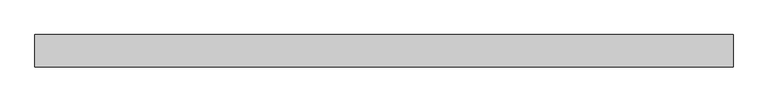
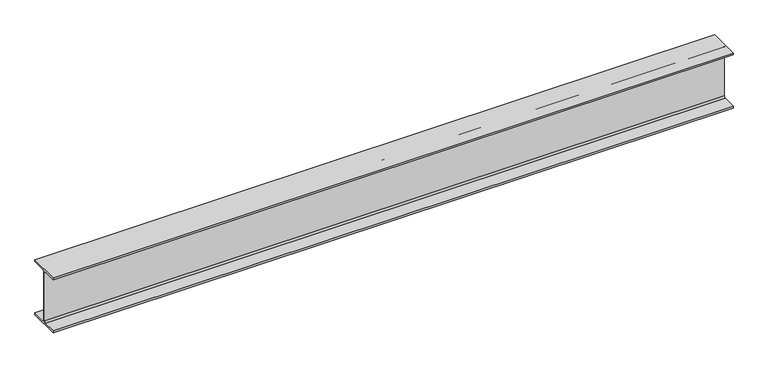
"""IFC4 building model written with IfcOpenShell, lengths in millimetres: beam geometry, Old_Steel Beam_H-KSD3502 : H_SB_ASB_H-200×200x8x12."""

import ifcopenshell
import ifcopenshell.guid

model = None  # the IFC model being written
_history = None  # IfcOwnerHistory: only IFC2X3 demands one
_inside = {}  # id of a spatial element -> (the spatial element, [elements in it])
_under = {}  # id of a project, library or spatial element -> (it, [spatial elements below it])
_declared = {}  # id of a project -> (the project, [libraries it declares])
_typed = {}  # id of a type object -> (the type object, [elements of that type])
_made_of = {}  # id of a material, layer set ... -> (it, [elements and type objects made of it])


def new_model(schema):
    """Start an empty IFC model of exactly this schema.

    Asked for "IFC4X3", IfcOpenShell would pick the latest addendum, in which some entities
    have other attributes; the version numbers below select the first issue.
    IFC2X3 requires an IfcOwnerHistory on every rooted entity: one is made here for all.
    """
    global model, _history
    if schema == "IFC4X3":
        model = ifcopenshell.file(schema_version=(4, 3, 0, 0))
    else:
        model = ifcopenshell.file(schema=schema)
    _inside.clear()
    _under.clear()
    _declared.clear()
    _typed.clear()
    _made_of.clear()
    _history = None
    if model.schema == "IFC2X3":
        org = make("IfcOrganization", Name="unknown")
        user = make(
            "IfcPersonAndOrganization",
            ThePerson=make("IfcPerson", FamilyName="unknown"),
            TheOrganization=org,
        )
        app = make(
            "IfcApplication",
            ApplicationDeveloper=org,
            Version="unknown",
            ApplicationFullName="unknown",
            ApplicationIdentifier="unknown",
        )
        _history = make(
            "IfcOwnerHistory",
            OwningUser=user,
            OwningApplication=app,
            ChangeAction="ADDED",
            CreationDate=0,
        )
    return model


def make(cls, **values):
    """One entity of the class cls with the attributes given. An attribute that is None is left unset."""
    return model.create_entity(
        cls, **{name: value for name, value in values.items() if value is not None}
    )


def rooted(cls, **values):
    """An entity with a GlobalId (a new one), such as an element, a storey or a relation."""
    return make(cls, GlobalId=ifcopenshell.guid.new(), OwnerHistory=_history, **values)


def si_unit(unit_type, name, prefix=None):
    """IfcSIUnit, for example si_unit("LENGTHUNIT", "METRE", prefix="MILLI")."""
    return make("IfcSIUnit", UnitType=unit_type, Prefix=prefix, Name=name)


def assignment(units):
    """IfcUnitAssignment: the units of a project."""
    return None if units is None else make("IfcUnitAssignment", Units=units)


def point(xyz):
    """IfcCartesianPoint."""
    return None if xyz is None else make("IfcCartesianPoint", Coordinates=xyz)


def direction(xyz):
    """IfcDirection."""
    return None if xyz is None else make("IfcDirection", DirectionRatios=xyz)


def frame(location, z_axis=None, x_axis=None):
    """IfcAxis2Placement3D, a coordinate frame: its origin and axes. An axis left out is left unset."""
    return make(
        "IfcAxis2Placement3D",
        Location=point(location),
        Axis=direction(z_axis),
        RefDirection=direction(x_axis),
    )


def frame_2d(location, x_axis=None):
    """IfcAxis2Placement2D, a coordinate frame in the plane: its origin and x axis."""
    return make(
        "IfcAxis2Placement2D", Location=point(location), RefDirection=direction(x_axis)
    )


def origin():
    """The frame at (0, 0, 0) with its axes left unset."""
    return frame((0.0, 0.0, 0.0))


def place(relative_to, where):
    """IfcLocalPlacement: puts the frame where relative to a parent placement (None: the world)."""
    return make(
        "IfcLocalPlacement", PlacementRelTo=relative_to, RelativePlacement=where
    )


def context(
    kind, dimensions, precision=None, world=None, true_north=None, identifier=None
):
    """IfcGeometricRepresentationContext, for example the 3D "Model" context."""
    return make(
        "IfcGeometricRepresentationContext",
        ContextIdentifier=identifier,
        ContextType=kind,
        CoordinateSpaceDimension=dimensions,
        Precision=precision,
        WorldCoordinateSystem=world,
        TrueNorth=true_north,
    )


def project(units=None, contexts=None):
    """IfcProject with its units and contexts."""
    return rooted(
        "IfcProject",
        Name="project",
        RepresentationContexts=contexts,
        UnitsInContext=assignment(units),
    )


def spatial(cls, under=None, at=None, **own):
    """A site, building, storey or space (cls), placed at a placement, below another one or the project."""
    s = rooted(cls, ObjectPlacement=at, **own)
    if under is not None:
        _under.setdefault(under.id(), (under, []))[1].append(s)
    return s


def polyline(points):
    """IfcPolyline through the points."""
    return make("IfcPolyline", Points=[point(p) for p in points])


def circle_curve(where, radius):
    """IfcCircle in the frame where."""
    return make("IfcCircle", Position=where, Radius=radius)


def trimmed(basis, trim1, trim2, sense, master):
    """IfcTrimmedCurve: the piece of a basis curve between two trims."""
    return make(
        "IfcTrimmedCurve",
        BasisCurve=basis,
        Trim1=trim1,
        Trim2=trim2,
        SenseAgreement=sense,
        MasterRepresentation=master,
    )


def segment(curve, same_sense, transition):
    """IfcCompositeCurveSegment."""
    return make(
        "IfcCompositeCurveSegment",
        Transition=transition,
        SameSense=same_sense,
        ParentCurve=curve,
    )


def composite_curve(segments, self_intersect=None):
    """IfcCompositeCurve: segments joined end to end."""
    return make("IfcCompositeCurve", Segments=segments, SelfIntersect=self_intersect)


def outline(outer, holes=None, kind="AREA"):
    """IfcArbitraryClosedProfileDef: a profile drawn as a closed curve; with holes, ...WithVoids."""
    if holes is None:
        return make("IfcArbitraryClosedProfileDef", ProfileType=kind, OuterCurve=outer)
    return make(
        "IfcArbitraryProfileDefWithVoids",
        ProfileType=kind,
        OuterCurve=outer,
        InnerCurves=holes,
    )


def extrude(swept, where, along, depth):
    """IfcExtrudedAreaSolid: the profile swept, set in the frame where, extruded along a direction by depth."""
    return make(
        "IfcExtrudedAreaSolid",
        SweptArea=swept,
        Position=where,
        ExtrudedDirection=direction(along),
        Depth=depth,
    )


def shape(context_of_items, identifier, shape_type, items):
    """IfcShapeRepresentation: the items that make up one representation, for example the "Body"."""
    return make(
        "IfcShapeRepresentation",
        ContextOfItems=context_of_items,
        RepresentationIdentifier=identifier,
        RepresentationType=shape_type,
        Items=items,
    )


def source(mapping_origin, context_of_items, identifier, shape_type, items):
    """IfcRepresentationMap: a shape defined once, which mapped items show again and again."""
    return make(
        "IfcRepresentationMap",
        MappingOrigin=mapping_origin,
        MappedRepresentation=shape(context_of_items, identifier, shape_type, items),
    )


def transform(
    local_origin,
    x_axis=None,
    y_axis=None,
    z_axis=None,
    scale=None,
    scale2=None,
    scale3=None,
    uniform=True,
):
    """IfcCartesianTransformationOperator3D, or its non-uniform kind. x_axis, y_axis, z_axis: its Axis1, 2, 3."""
    if uniform:
        return make(
            "IfcCartesianTransformationOperator3D",
            Axis1=direction(x_axis),
            Axis2=direction(y_axis),
            LocalOrigin=point(local_origin),
            Scale=scale,
            Axis3=direction(z_axis),
        )
    return make(
        "IfcCartesianTransformationOperator3DnonUniform",
        Axis1=direction(x_axis),
        Axis2=direction(y_axis),
        LocalOrigin=point(local_origin),
        Scale=scale,
        Axis3=direction(z_axis),
        Scale2=scale2,
        Scale3=scale3,
    )


def mapped(mapping_source, mapping_target):
    """IfcMappedItem: shows the shape of a source again, moved by a transform."""
    return make(
        "IfcMappedItem", MappingSource=mapping_source, MappingTarget=mapping_target
    )


def made_of(thing, what):
    """Note that an element or type object is made of a material, layer set ...; save() writes the relation."""
    if what is not None:
        _made_of.setdefault(what.id(), (what, []))[1].append(thing)
    return thing


def element(
    cls,
    number,
    at=None,
    inside=None,
    cuts=None,
    type_object=None,
    material=None,
    context=None,
    identifier="Body",
    shape_type=None,
    held_by="IfcProductDefinitionShape",
    body=None,
    shapes=None,
    **own,
):
    """One element of the class cls, such as IfcWall. Its Tag is "e" and its number.

    at: its placement. inside: the storey or other place that contains it. cuts: it is an
    opening in that element (IfcRelVoidsElement). A single representation is given by context,
    identifier, shape_type and body (its items); several are given by shapes. held_by: the class
    of the entity that holds the representations. save() writes the other relations.
    """
    e = rooted(cls, Tag="e%d" % number, ObjectPlacement=at, **own)
    if body is not None:
        shapes = [shape(context, identifier, shape_type, body)]
    if shapes is not None:
        e.Representation = make(held_by, Representations=shapes)
    if inside is not None:
        _inside.setdefault(inside.id(), (inside, []))[1].append(e)
    if cuts is not None:
        rooted(
            "IfcRelVoidsElement", RelatingBuildingElement=cuts, RelatedOpeningElement=e
        )
    if type_object is not None:
        _typed.setdefault(type_object.id(), (type_object, []))[1].append(e)
    return made_of(e, material)


def aggregate(whole, parts):
    """IfcRelAggregates: a whole, such as a stair, and the parts it consists of."""
    return rooted("IfcRelAggregates", RelatingObject=whole, RelatedObjects=parts)


def save(model, path):
    """Write the relations noted so far, then the file.

    IfcRelAggregates (storeys below a building ...), IfcRelContainedInSpatialStructure (elements
    in a storey), IfcRelDefinesByType, IfcRelAssociatesMaterial and IfcRelDeclares: one each for
    every whole, place, type object, material and project.
    """
    for whole, parts in _under.values():
        aggregate(whole, parts)
    for where, things in _inside.values():
        rooted(
            "IfcRelContainedInSpatialStructure",
            RelatedElements=things,
            RelatingStructure=where,
        )
    for kind, things in _typed.values():
        rooted("IfcRelDefinesByType", RelatedObjects=things, RelatingType=kind)
    for what, things in _made_of.values():
        rooted("IfcRelAssociatesMaterial", RelatedObjects=things, RelatingMaterial=what)
    for by, libraries in _declared.values():
        rooted("IfcRelDeclares", RelatingContext=by, RelatedDefinitions=libraries)
    model.write(path)


def beam_588beb59(model_context):
    return source(origin(), model_context, "Body", "SweptSolid", [
        extrude(outline(composite_curve([segment(polyline([(82.5, -141.5), (82.5, -151.7), (-82.5, -151.7), (-82.5, -141.5), (-11.9, -141.5)]), True, "CONTINUOUS"), segment(trimmed(circle_curve(frame_2d((-11.9, -132.6)), 8.9), [point((-11.9, -141.5))], [point((-3.0, -132.6))], True, "CARTESIAN"), True, "CONTINUOUS"), segment(polyline([(-3.0, -132.6), (-3.0, 132.6)]), True, "CONTINUOUS"), segment(trimmed(circle_curve(frame_2d((-11.9, 132.6)), 8.9), [point((-3.0, 132.6))], [point((-11.9, 141.5))], True, "CARTESIAN"), True, "CONTINUOUS"), segment(polyline([(-11.9, 141.5), (-82.5, 141.5), (-82.5, 151.7), (82.5, 151.7), (82.5, 141.5), (11.9, 141.5)]), True, "CONTINUOUS"), segment(trimmed(circle_curve(frame_2d((11.9, 132.6)), 8.9), [point((11.9, 141.5))], [point((3.0, 132.6))], True, "CARTESIAN"), True, "CONTINUOUS"), segment(polyline([(3.0, 132.6), (3.0, -132.6)]), True, "CONTINUOUS"), segment(trimmed(circle_curve(frame_2d((11.9, -132.6)), 8.9), [point((3.0, -132.6))], [point((11.9, -141.5))], True, "CARTESIAN"), True, "CONTINUOUS"), segment(polyline([(11.9, -141.5), (82.5, -141.5)]), True, "CONTINUOUS")], self_intersect=False)), frame((-1835.8461272, 0.0, 0.0), z_axis=(1.0, 0.0, 0.0), x_axis=(0.0, 1.0, 0.0)), (0.0, 0.0, 1.0), 3545.7762812),
    ])


if __name__ == "__main__":
    model = new_model("IFC4")
    model_context = context("Model", 3, world=origin())
    ifc_project = project(units=[si_unit("LENGTHUNIT", "METRE", prefix="MILLI")], contexts=[model_context])
    site = spatial("IfcSite", under=ifc_project)
    building = spatial("IfcBuilding", under=site)
    placement = place(None, origin())
    beam_shape = beam_588beb59(model_context)
    element("IfcBeam", 1, ObjectType="Old_Steel Beam_H-KSD3502 : H_SB_ASB_H-200×200x8x12", at=placement, inside=building, context=model_context, shape_type="MappedRepresentation", body=[
        mapped(beam_shape, transform((0.0, 0.0, 0.0), x_axis=(1.0, 0.0, 0.0), y_axis=(0.0, 1.0, 0.0), z_axis=(0.0, 0.0, 1.0))),
    ])
    save(model, "model.ifc")

# Revit data of these elements
# Type "Old_Steel Beam_H-KSD3502 : H_SB_ASB_H-200×200x8x12"
#   Width = 20.0 cm
#   Web Thickness = 0.8 cm
#   Web Fillet = 1.3 cm
#   Warping Constant = 141376.0 cm⁶
#   Torsional Moment of Inertia = 26.2485 cm⁴
#   Torsional Modulus = 1.0 cm³
#   Section Area = 63.53 cm²
#   Plastic Modulus weak axis = 244.0 cm³
#   Plastic Modulus strong axis = 525.0 cm³
#   Perimeter = 1.16 m²/m
#   Nominal Weight = 49.90 kgf/m
#   Moment of Inertia weak axis = 1600.00 cm⁴
#   Moment of Inertia strong axis = 4720.00 cm⁴
#   Height = 20.0 cm
#   Flange Thickness = 1.2 cm
#   Elastic Modulus weak axis = 160.0 cm³
#   Elastic Modulus strong axis = 472.0 cm³
#   Centroid Vertical = 10.0 cm
#   Centroid Horizontal = 10.0 cm
#   Length [instance default] = 1.5240 m
#   Structural Material [instance default] = Steel, 45-345
#   Assembly Code = ""
# Element 1 (IfcBeam, "Old_Steel Beam_H-KSD3502 : H_SB_ASB_H-200×200x8x12")
#   Structural Material = none
# Materials
#   "Steel, 45-345": class "Metal", colour RGB 189 187 185, transparency 0, Description = "Steel 345 MPa", Cost = 0
